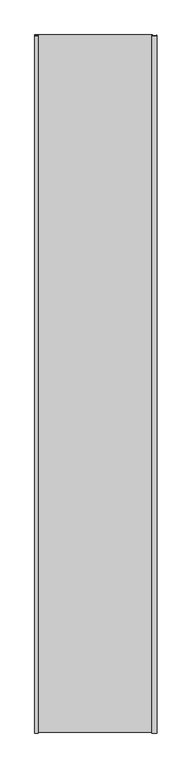
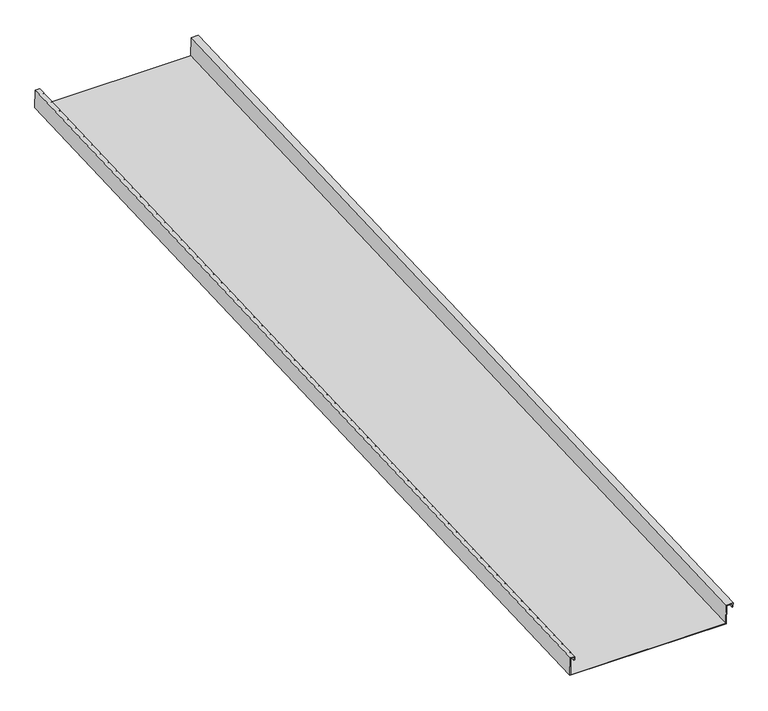
"""IFC4 building model written with IfcOpenShell, lengths in millimetres: proxy geometry, Generic Models 2:Generic Models 2:310765:Generic Models 2:310765 : Generic Models 2:Generic Models 2:310765:62 : Generic Models 2:Generic Models 2:310765:Generic Models 2:310765 : Generic Models 2:Generic Models 2:310765:300385."""

from ifc_helpers import new_model, si_unit, frame, origin, place, context, project, spatial, polyline, outline, extrude, source, transform, mapped, element, save


def generic_models_3232bfe8(model_context):
    return source(origin(), model_context, "Body", "SweptSolid", [
        extrude(outline(polyline([(50.8, 0.0), (50.8, 14.2875), (41.275, 14.2875), (41.275, 15.875), (52.3874999, 15.875), (52.3874999, -1.5875), (1.5874999, -1.5875), (1.5874999, -404.8125), (47.625, -404.8125), (47.625, -396.875), (39.6875, -396.875), (39.6875, -395.2875), (49.2124999, -395.2875), (49.2124999, -406.4), (0.0, -406.4), (0.0, 0.0), (50.8, 0.0)])), frame((580020.2953039, -581447.5605462, 3847.9454697), z_axis=(0.0, 0.9991330730923567, 0.04163054471206783), x_axis=(0.0, -0.04163054471206783, 0.9991330730923567)), (0.0, 0.0, 1.0), 2407.4486947),
    ])


if __name__ == "__main__":
    model = new_model("IFC4")
    model_context = context("Model", 3, world=origin())
    ifc_project = project(units=[si_unit("LENGTHUNIT", "METRE", prefix="MILLI")], contexts=[model_context])
    site = spatial("IfcSite", under=ifc_project)
    building = spatial("IfcBuilding", under=site)
    placement = place(None, origin())
    generic_models_shape = generic_models_3232bfe8(model_context)
    element("IfcBuildingElementProxy", 1, Name="Generic Models 2:Generic Models 2:310765:Generic Models 2:310765 : Generic Models 2:Generic Models 2:310765:62 : Generic Models 2:Generic Models 2:310765:Generic Models 2:310765 : Generic Models 2:Generic Models 2:310765:300385", ObjectType="Generic Models 2:Generic Models 2:310765:Generic Models 2:310765 : Generic Models 2:Generic Models 2:310765:62 : Generic Models 2:Generic Models 2:310765:Generic Models 2:310765 : Generic Models 2:Generic Models 2:310765:300385", at=placement, inside=building, context=model_context, shape_type="MappedRepresentation", body=[
        mapped(generic_models_shape, transform((0.0, 0.0, 0.0), x_axis=(1.0, 0.0, 0.0), y_axis=(0.0, 1.0, 0.0), z_axis=(0.0, 0.0, 1.0))),
    ])
    save(model, "model.ifc")

# Revit data of these elements
# Type "Generic Models 2:Generic Models 2:310765:Generic Models 2:310765 : Generic Models 2:Generic Models 2:310765:62 : Generic Models 2:Generic Models 2:310765:Generic Models 2:310765 : Generic Models 2:Generic Models 2:310765:300385"
#   NameOverride = "Generic Models 2:Generic Models 2:310765:Generic Models 2:310765 : Generic Models 2:Generic Models 2:310765:300385"
#   ObjectTypeOverride = "Generic Models 2:310765 : Generic Models 2:Generic Models 2:310765"
#   Reference = "Generic Models 2"
#   Tag = "300385"
# Element 1 (IfcBuildingElementProxy, "Generic Models 2:Generic Models 2:310765:Generic Models 2:310765 : Generic Models 2:Generic Models 2:310765:62 : Generic Models 2:Generic Models 2:310765:Generic Models 2:310765 : Generic Models 2:Generic Models 2:310765:300385")
#   Materials on its faces: "THERMAL BROKEN ALUMINUM STOREFRONT FOR POLYCARBONATE"
# Materials
#   "THERMAL BROKEN ALUMINUM STOREFRONT FOR POLYCARBONATE": class "Unassigned", colour RGB 244 244 244, transparency 0, Keynote = "M07611300.01", Cost = 0
